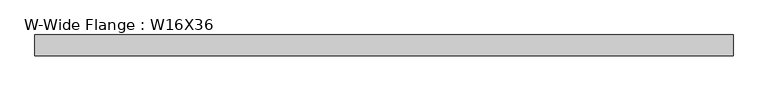
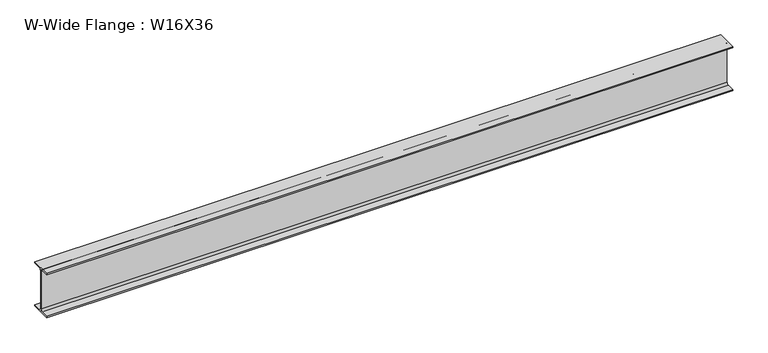
"""IFC4 building model written with IfcOpenShell, lengths in millimetres: beam geometry, W-Wide Flange : W16X36."""

from ifc_helpers import new_model, si_unit, point, frame, frame_2d, origin, place, context, project, spatial, polyline, circle_curve, trimmed, segment, composite_curve, outline, extrude, source, transform, mapped, element, save


def w_wide_flange_w16x36_8371616b(model_context):
    return source(origin(), model_context, "Body", "SweptSolid", [
        extrude(outline(composite_curve([segment(polyline([(88.773, -191.008), (88.773, -201.93), (-88.773, -201.93), (-88.773, -191.008), (-21.3995, -191.008)]), True, "CONTINUOUS"), segment(trimmed(circle_curve(frame_2d((-21.3995, -173.355)), 17.653), [point((-21.3995, -191.008))], [point((-3.7465, -173.355))], True, "CARTESIAN"), True, "CONTINUOUS"), segment(polyline([(-3.7465, -173.355), (-3.7465, 173.355)]), True, "CONTINUOUS"), segment(trimmed(circle_curve(frame_2d((-21.3995, 173.355)), 17.653), [point((-3.7465, 173.355))], [point((-21.3995, 191.008))], True, "CARTESIAN"), True, "CONTINUOUS"), segment(polyline([(-21.3995, 191.008), (-88.773, 191.008), (-88.773, 201.93), (88.773, 201.93), (88.773, 191.008), (21.3995, 191.008)]), True, "CONTINUOUS"), segment(trimmed(circle_curve(frame_2d((21.3995, 173.355)), 17.653), [point((21.3995, 191.008))], [point((3.7465, 173.355))], True, "CARTESIAN"), True, "CONTINUOUS"), segment(polyline([(3.7465, 173.355), (3.7465, -173.355)]), True, "CONTINUOUS"), segment(trimmed(circle_curve(frame_2d((21.3995, -173.355)), 17.653), [point((3.7465, -173.355))], [point((21.3995, -191.008))], True, "CARTESIAN"), True, "CONTINUOUS"), segment(polyline([(21.3995, -191.008), (88.773, -191.008)]), True, "CONTINUOUS")], self_intersect=False)), frame((-2904.3981568, 0.0, 0.0), z_axis=(1.0, 0.0, 0.0), x_axis=(0.0, 1.0, 0.0)), (0.0, 0.0, 1.0), 5935.7963136),
    ])


if __name__ == "__main__":
    model = new_model("IFC4")
    model_context = context("Model", 3, world=origin())
    ifc_project = project(units=[si_unit("LENGTHUNIT", "METRE", prefix="MILLI")], contexts=[model_context])
    site = spatial("IfcSite", under=ifc_project)
    building = spatial("IfcBuilding", under=site)
    placement = place(None, origin())
    w_wide_flange_w16x36_shape = w_wide_flange_w16x36_8371616b(model_context)
    element("IfcBeam", 1, ObjectType="W-Wide Flange : W16X36", at=placement, inside=building, context=model_context, shape_type="MappedRepresentation", body=[
        mapped(w_wide_flange_w16x36_shape, transform((0.0, 0.0, 0.0), x_axis=(1.0, 0.0, 0.0), y_axis=(0.0, 1.0, 0.0), z_axis=(0.0, 0.0, 1.0))),
    ])
    save(model, "model.ifc")

# Revit data of these elements
# Type "W-Wide Flange : W16X36"
#   Assembly Code = "B10"
#   W = 36
#   Length [instance default] = 5' - 0"
#   bf = 0' - 6.99"
#   d = 1' - 3.9"
#   k = 0' - 1 1/8"
#   k2 = 0' - 0.695"
#   tf = 0' - 0.43"
#   tw = 0' - 0.295"
#   A = 0.0736111 SF
#   Structural Material [instance default] = Steel ASTM A992
# Element 1 (IfcBeam, "W-Wide Flange : W16X36")
#   Materials on its faces: "Steel ASTM A992"
# Materials
#   "Steel ASTM A992": class "Metal", colour RGB 199 199 199, transparency 0, Description = "Structural steel 50ksi", Cost = 0
